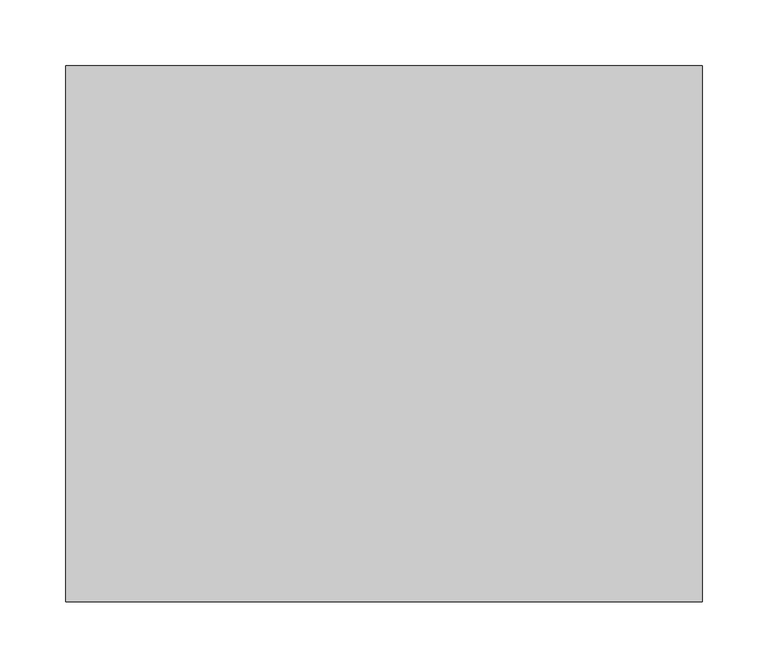
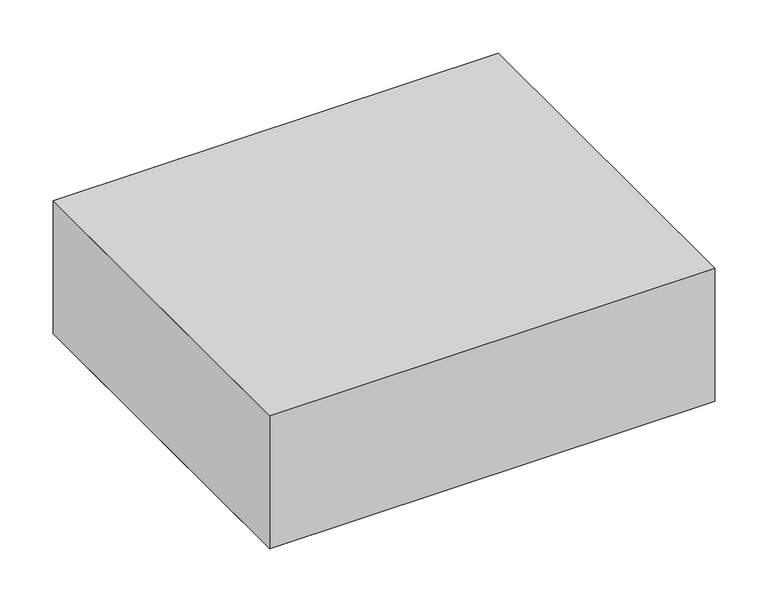
"""IFC4 building model written with IfcOpenShell, lengths in millimetres: proxy geometry, M3175 - Electrosurgical Unit, Dual Output : M3175 - Electrosurgical Unit, Dual Output."""

from ifc_helpers import new_model, si_unit, origin, origin_with_axes, place, context, project, spatial, polyline, outline, extrude, source, transform, mapped, element, save


def specialty_equipment_c6880412(model_context):
    return source(origin(), model_context, "Body", "SweptSolid", [
        extrude(outline(polyline([(241.3, 203.2), (241.3, -203.2), (-241.3, -203.2), (-241.3, 203.2), (241.3, 203.2)])), origin_with_axes(), (0.0, 0.0, 1.0), 152.4),
        extrude(outline(polyline([(-241.3, 203.2), (241.3, 203.2), (241.3, -203.2), (-241.3, -203.2), (-241.3, 0.0), (-241.3, 203.2)])), origin_with_axes(), (0.0, 0.0, 1.0), 152.4),
    ])


if __name__ == "__main__":
    model = new_model("IFC4")
    model_context = context("Model", 3, world=origin())
    ifc_project = project(units=[si_unit("LENGTHUNIT", "METRE", prefix="MILLI")], contexts=[model_context])
    site = spatial("IfcSite", under=ifc_project)
    building = spatial("IfcBuilding", under=site)
    placement = place(None, origin())
    specialty_equipment_shape = specialty_equipment_c6880412(model_context)
    element("IfcBuildingElementProxy", 1, Name="M3175 - Electrosurgical Unit, Dual Output : M3175 - Electrosurgical Unit, Dual Output", ObjectType="M3175 - Electrosurgical Unit, Dual Output : M3175 - Electrosurgical Unit, Dual Output", at=placement, inside=building, context=model_context, shape_type="MappedRepresentation", body=[
        mapped(specialty_equipment_shape, transform((0.0, 0.0, 0.0), x_axis=(1.0, 0.0, 0.0), y_axis=(0.0, 1.0, 0.0), z_axis=(0.0, 0.0, 1.0))),
    ])
    save(model, "model.ifc")

# Revit data of these elements
# Type "M3175 - Electrosurgical Unit, Dual Output : M3175 - Electrosurgical Unit, Dual Output"
#   Watts2 = "0"
#   Watts1 = "480"
#   Unit_Issue = "EA"
#   UTIL_6_Misc = "-"
#   UTIL_5_NonMedGas = "-"
#   UTIL_4_MiscGas = "-"
#   UTIL_3_MedGas = "-"
#   UTIL_2_Elec = "A"
#   UTIL_1_WaterDrain = "-"
#   Nomenclature = "Electrosurgical Unit, Dual Output"
#   NSN = "6515"
#   Location [instance default] = ""
#   JSN = "M3175"
#   Fund_Source_VA = "-"
#   Fund_Source_Navy = "-"
#   Fund_Source_Army = "-"
#   Fund_Source_AF = "-"
#   ELEC_Volts2 = "0"
#   ELEC_Volts1 = "120"
#   ELEC_Phase2 = "0"
#   ELEC_Phase1 = "1"
#   ELEC_HertzSwitch = "0"
#   ELEC_HertzDependent = "1"
#   ELEC_Hertz = "60"
#   ELEC_Amps2 = "0"
#   ELEC_Amps1 = "4"
#   DetailDescription = "Dual output electrosurgical unit. Solid state power source with foot switch jacks, monopolar and bipolar outputs, and four independent modes of operation. Used in the operating room or surgicenter as an alternative to the scalpel for cutting tissue."
#   CAT_VA = "C"
#   CAT_Navy = "C"
#   CAT_IHS = "-"
#   CAT_Army = "C"
#   CAT_AF = "C"
#   BTUperhour = "0"
#   Weight_IP = 34
#   DIM_Width_IP = 1' - 7"
#   DIM_Height_IP = 0' - 6"
#   DIM_Depth_IP = 1' - 4"
# Element 1 (IfcBuildingElementProxy, "M3175 - Electrosurgical Unit, Dual Output : M3175 - Electrosurgical Unit, Dual Output")
#   Location = "ORGS1"
#   Materials on its faces: "EquipSpace"
# Materials
#   "EquipSpace": class "Unassigned", colour RGB 221 217 195, transparency 0.5
